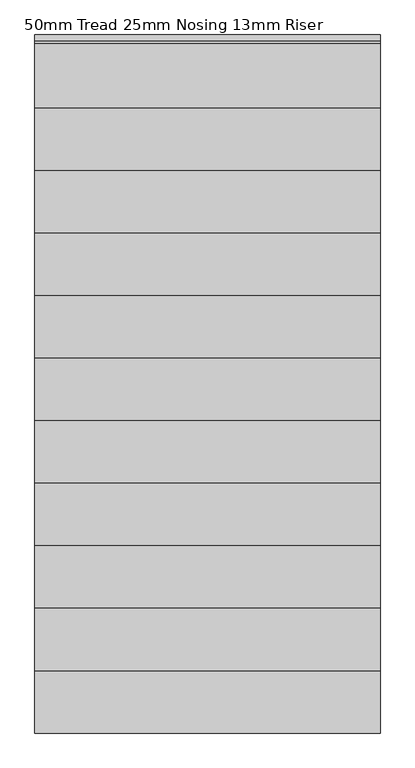
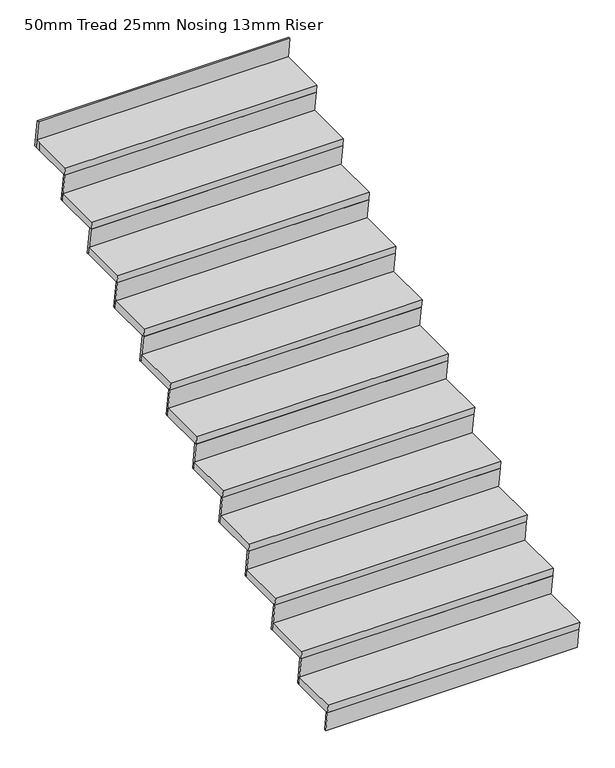
"""IFC4 building model written with IfcOpenShell, lengths in millimetres: stair flight geometry, 50mm Tread 25mm Nosing 13mm Riser."""

from ifc_helpers import new_model, si_unit, origin, place, context, project, spatial, faceted_brep, source, transform, mapped, element, save


def stair_flight_50mm_tread_25mm_nosing_13mm_riser_3e0063ee(model_context):
    return source(origin(), model_context, "Body", "Brep", [
        faceted_brep([(-499.4393676, 4584.7509075, 15676.4705882), (-499.4393676, 4591.8342409, 15626.4705882), (-2019.4393676, 4591.8342409, 15626.4705882), (-2019.4393676, 4584.7509075, 15676.4705882), (-2019.4393676, 4284.7509075, 15676.4705882), (-499.4393676, 4284.7509075, 15676.4705882), (-499.4393676, 4291.8342409, 15626.4705882), (-2019.4393676, 4291.8342409, 15626.4705882)], [[[0, 1, 2, 3]], [[3, 4, 5, 0]], [[2, 1, 6, 7]], [[4, 3, 2, 7]], [[0, 5, 6, 1]], [[5, 4, 7, 6]]]),
        faceted_brep([(-499.4393676, 4291.8342409, 15626.4705882), (-499.4393676, 4309.7509075, 15500.0), (-499.4393676, 4322.3757185, 15500.0), (-499.4393676, 4304.4590518, 15626.4705882), (-2019.4393676, 4291.8342409, 15626.4705882), (-2019.4393676, 4304.4590518, 15626.4705882), (-2019.4393676, 4322.3757185, 15500.0), (-2019.4393676, 4309.7509075, 15500.0)], [[[0, 1, 2, 3]], [[4, 5, 6, 7]], [[1, 0, 4, 7]], [[2, 1, 7, 6]], [[3, 2, 6, 5]], [[0, 3, 5, 4]]]),
        faceted_brep([(-499.4393676, 4566.8342409, 15802.9411765), (-499.4393676, 4591.8342409, 15626.4705882), (-499.4393676, 4604.4590518, 15626.4705882), (-499.4393676, 4579.4590518, 15802.9411765), (-2019.4393676, 4566.8342409, 15802.9411765), (-2019.4393676, 4579.4590518, 15802.9411765), (-2019.4393676, 4604.4590518, 15626.4705882), (-2019.4393676, 4591.8342409, 15626.4705882)], [[[0, 1, 2, 3]], [[4, 5, 6, 7]], [[1, 0, 4, 7]], [[2, 1, 7, 6]], [[3, 2, 6, 5]], [[0, 3, 5, 4]]]),
        faceted_brep([(-2019.4393676, 4859.7509075, 15852.9411765), (-2019.4393676, 4559.7509075, 15852.9411765), (-499.4393676, 4559.7509075, 15852.9411765), (-499.4393676, 4859.7509075, 15852.9411765), (-2019.4393676, 4866.8342409, 15802.9411765), (-499.4393676, 4866.8342409, 15802.9411765), (-499.4393676, 4566.8342409, 15802.9411765), (-2019.4393676, 4566.8342409, 15802.9411765)], [[[0, 1, 2, 3]], [[4, 5, 6, 7]], [[1, 0, 4, 7]], [[3, 2, 6, 5]], [[3, 5, 4, 0]], [[2, 1, 7, 6]]]),
        faceted_brep([(-499.4393676, 4841.8342409, 15979.4117647), (-499.4393676, 4866.8342409, 15802.9411765), (-499.4393676, 4879.4590518, 15802.9411765), (-499.4393676, 4854.4590518, 15979.4117647), (-2019.4393676, 4841.8342409, 15979.4117647), (-2019.4393676, 4854.4590518, 15979.4117647), (-2019.4393676, 4879.4590518, 15802.9411765), (-2019.4393676, 4866.8342409, 15802.9411765)], [[[0, 1, 2, 3]], [[4, 5, 6, 7]], [[1, 0, 4, 7]], [[2, 1, 7, 6]], [[3, 2, 6, 5]], [[0, 3, 5, 4]]]),
        faceted_brep([(-2019.4393676, 5134.7509075, 16029.4117647), (-2019.4393676, 4834.7509075, 16029.4117647), (-499.4393676, 4834.7509075, 16029.4117647), (-499.4393676, 5134.7509075, 16029.4117647), (-2019.4393676, 5141.8342409, 15979.4117647), (-499.4393676, 5141.8342409, 15979.4117647), (-499.4393676, 4841.8342409, 15979.4117647), (-2019.4393676, 4841.8342409, 15979.4117647)], [[[0, 1, 2, 3]], [[4, 5, 6, 7]], [[1, 0, 4, 7]], [[3, 2, 6, 5]], [[3, 5, 4, 0]], [[2, 1, 7, 6]]]),
        faceted_brep([(-499.4393676, 5116.8342409, 16155.8823529), (-499.4393676, 5141.8342409, 15979.4117647), (-499.4393676, 5154.4590518, 15979.4117647), (-499.4393676, 5129.4590518, 16155.8823529), (-2019.4393676, 5116.8342409, 16155.8823529), (-2019.4393676, 5129.4590518, 16155.8823529), (-2019.4393676, 5154.4590518, 15979.4117647), (-2019.4393676, 5141.8342409, 15979.4117647)], [[[0, 1, 2, 3]], [[4, 5, 6, 7]], [[1, 0, 4, 7]], [[2, 1, 7, 6]], [[3, 2, 6, 5]], [[0, 3, 5, 4]]]),
        faceted_brep([(-2019.4393676, 5409.7509075, 16205.8823529), (-2019.4393676, 5109.7509075, 16205.8823529), (-499.4393676, 5109.7509075, 16205.8823529), (-499.4393676, 5409.7509075, 16205.8823529), (-2019.4393676, 5416.8342409, 16155.8823529), (-499.4393676, 5416.8342409, 16155.8823529), (-499.4393676, 5116.8342409, 16155.8823529), (-2019.4393676, 5116.8342409, 16155.8823529)], [[[0, 1, 2, 3]], [[4, 5, 6, 7]], [[1, 0, 4, 7]], [[3, 2, 6, 5]], [[3, 5, 4, 0]], [[2, 1, 7, 6]]]),
        faceted_brep([(-499.4393676, 5391.8342409, 16332.3529412), (-499.4393676, 5416.8342409, 16155.8823529), (-499.4393676, 5429.4590518, 16155.8823529), (-499.4393676, 5404.4590518, 16332.3529412), (-2019.4393676, 5391.8342409, 16332.3529412), (-2019.4393676, 5404.4590518, 16332.3529412), (-2019.4393676, 5429.4590518, 16155.8823529), (-2019.4393676, 5416.8342409, 16155.8823529)], [[[0, 1, 2, 3]], [[4, 5, 6, 7]], [[1, 0, 4, 7]], [[2, 1, 7, 6]], [[3, 2, 6, 5]], [[0, 3, 5, 4]]]),
        faceted_brep([(-2019.4393676, 5684.7509075, 16382.3529412), (-2019.4393676, 5384.7509075, 16382.3529412), (-499.4393676, 5384.7509075, 16382.3529412), (-499.4393676, 5684.7509075, 16382.3529412), (-2019.4393676, 5691.8342409, 16332.3529412), (-499.4393676, 5691.8342409, 16332.3529412), (-499.4393676, 5391.8342409, 16332.3529412), (-2019.4393676, 5391.8342409, 16332.3529412)], [[[0, 1, 2, 3]], [[4, 5, 6, 7]], [[1, 0, 4, 7]], [[3, 2, 6, 5]], [[3, 5, 4, 0]], [[2, 1, 7, 6]]]),
        faceted_brep([(-499.4393676, 5666.8342409, 16508.8235294), (-499.4393676, 5691.8342409, 16332.3529412), (-499.4393676, 5704.4590518, 16332.3529412), (-499.4393676, 5679.4590518, 16508.8235294), (-2019.4393676, 5666.8342409, 16508.8235294), (-2019.4393676, 5679.4590518, 16508.8235294), (-2019.4393676, 5704.4590518, 16332.3529412), (-2019.4393676, 5691.8342409, 16332.3529412)], [[[0, 1, 2, 3]], [[4, 5, 6, 7]], [[1, 0, 4, 7]], [[2, 1, 7, 6]], [[3, 2, 6, 5]], [[0, 3, 5, 4]]]),
        faceted_brep([(-2019.4393676, 5959.7509075, 16558.8235294), (-2019.4393676, 5659.7509075, 16558.8235294), (-499.4393676, 5659.7509075, 16558.8235294), (-499.4393676, 5959.7509075, 16558.8235294), (-2019.4393676, 5966.8342409, 16508.8235294), (-499.4393676, 5966.8342409, 16508.8235294), (-499.4393676, 5666.8342409, 16508.8235294), (-2019.4393676, 5666.8342409, 16508.8235294)], [[[0, 1, 2, 3]], [[4, 5, 6, 7]], [[1, 0, 4, 7]], [[3, 2, 6, 5]], [[3, 5, 4, 0]], [[2, 1, 7, 6]]]),
        faceted_brep([(-499.4393676, 5941.8342409, 16685.2941176), (-499.4393676, 5966.8342409, 16508.8235294), (-499.4393676, 5979.4590518, 16508.8235294), (-499.4393676, 5954.4590518, 16685.2941176), (-2019.4393676, 5941.8342409, 16685.2941176), (-2019.4393676, 5954.4590518, 16685.2941176), (-2019.4393676, 5979.4590518, 16508.8235294), (-2019.4393676, 5966.8342409, 16508.8235294)], [[[0, 1, 2, 3]], [[4, 5, 6, 7]], [[1, 0, 4, 7]], [[2, 1, 7, 6]], [[3, 2, 6, 5]], [[0, 3, 5, 4]]]),
        faceted_brep([(-2019.4393676, 6234.7509075, 16735.2941176), (-2019.4393676, 5934.7509075, 16735.2941176), (-499.4393676, 5934.7509075, 16735.2941176), (-499.4393676, 6234.7509075, 16735.2941176), (-2019.4393676, 6241.8342409, 16685.2941176), (-499.4393676, 6241.8342409, 16685.2941176), (-499.4393676, 5941.8342409, 16685.2941176), (-2019.4393676, 5941.8342409, 16685.2941176)], [[[0, 1, 2, 3]], [[4, 5, 6, 7]], [[1, 0, 4, 7]], [[3, 2, 6, 5]], [[3, 5, 4, 0]], [[2, 1, 7, 6]]]),
        faceted_brep([(-499.4393676, 6216.8342409, 16861.7647059), (-499.4393676, 6241.8342409, 16685.2941176), (-499.4393676, 6254.4590518, 16685.2941176), (-499.4393676, 6229.4590518, 16861.7647059), (-2019.4393676, 6216.8342409, 16861.7647059), (-2019.4393676, 6229.4590518, 16861.7647059), (-2019.4393676, 6254.4590518, 16685.2941176), (-2019.4393676, 6241.8342409, 16685.2941176)], [[[0, 1, 2, 3]], [[4, 5, 6, 7]], [[1, 0, 4, 7]], [[2, 1, 7, 6]], [[3, 2, 6, 5]], [[0, 3, 5, 4]]]),
        faceted_brep([(-2019.4393676, 6509.7509075, 16911.7647059), (-2019.4393676, 6209.7509075, 16911.7647059), (-499.4393676, 6209.7509075, 16911.7647059), (-499.4393676, 6509.7509075, 16911.7647059), (-2019.4393676, 6516.8342409, 16861.7647059), (-499.4393676, 6516.8342409, 16861.7647059), (-499.4393676, 6216.8342409, 16861.7647059), (-2019.4393676, 6216.8342409, 16861.7647059)], [[[0, 1, 2, 3]], [[4, 5, 6, 7]], [[1, 0, 4, 7]], [[3, 2, 6, 5]], [[3, 5, 4, 0]], [[2, 1, 7, 6]]]),
        faceted_brep([(-499.4393676, 6491.8342409, 17038.2352941), (-499.4393676, 6516.8342409, 16861.7647059), (-499.4393676, 6529.4590518, 16861.7647059), (-499.4393676, 6504.4590518, 17038.2352941), (-2019.4393676, 6491.8342409, 17038.2352941), (-2019.4393676, 6504.4590518, 17038.2352941), (-2019.4393676, 6529.4590518, 16861.7647059), (-2019.4393676, 6516.8342409, 16861.7647059)], [[[0, 1, 2, 3]], [[4, 5, 6, 7]], [[1, 0, 4, 7]], [[2, 1, 7, 6]], [[3, 2, 6, 5]], [[0, 3, 5, 4]]]),
        faceted_brep([(-2019.4393676, 6784.7509075, 17088.2352941), (-2019.4393676, 6484.7509075, 17088.2352941), (-499.4393676, 6484.7509075, 17088.2352941), (-499.4393676, 6784.7509075, 17088.2352941), (-2019.4393676, 6791.8342409, 17038.2352941), (-499.4393676, 6791.8342409, 17038.2352941), (-499.4393676, 6491.8342409, 17038.2352941), (-2019.4393676, 6491.8342409, 17038.2352941)], [[[0, 1, 2, 3]], [[4, 5, 6, 7]], [[1, 0, 4, 7]], [[3, 2, 6, 5]], [[3, 5, 4, 0]], [[2, 1, 7, 6]]]),
        faceted_brep([(-499.4393676, 6766.8342409, 17214.7058824), (-499.4393676, 6791.8342409, 17038.2352941), (-499.4393676, 6804.4590518, 17038.2352941), (-499.4393676, 6779.4590518, 17214.7058824), (-2019.4393676, 6766.8342409, 17214.7058824), (-2019.4393676, 6779.4590518, 17214.7058824), (-2019.4393676, 6804.4590518, 17038.2352941), (-2019.4393676, 6791.8342409, 17038.2352941)], [[[0, 1, 2, 3]], [[4, 5, 6, 7]], [[1, 0, 4, 7]], [[2, 1, 7, 6]], [[3, 2, 6, 5]], [[0, 3, 5, 4]]]),
        faceted_brep([(-2019.4393676, 7059.7509075, 17264.7058824), (-2019.4393676, 6759.7509075, 17264.7058824), (-499.4393676, 6759.7509075, 17264.7058824), (-499.4393676, 7059.7509075, 17264.7058824), (-2019.4393676, 7066.8342409, 17214.7058824), (-499.4393676, 7066.8342409, 17214.7058824), (-499.4393676, 6766.8342409, 17214.7058824), (-2019.4393676, 6766.8342409, 17214.7058824)], [[[0, 1, 2, 3]], [[4, 5, 6, 7]], [[1, 0, 4, 7]], [[3, 2, 6, 5]], [[3, 5, 4, 0]], [[2, 1, 7, 6]]]),
        faceted_brep([(-499.4393676, 7316.8342409, 17567.6470588), (-499.4393676, 7341.8342409, 17391.1764706), (-499.4393676, 7354.4590518, 17391.1764706), (-499.4393676, 7329.4590518, 17567.6470588), (-2019.4393676, 7316.8342409, 17567.6470588), (-2019.4393676, 7329.4590518, 17567.6470588), (-2019.4393676, 7354.4590518, 17391.1764706), (-2019.4393676, 7341.8342409, 17391.1764706)], [[[0, 1, 2, 3]], [[4, 5, 6, 7]], [[1, 0, 4, 7]], [[2, 1, 7, 6]], [[3, 2, 6, 5]], [[0, 3, 5, 4]]]),
        faceted_brep([(-499.4393676, 7041.8342409, 17391.1764706), (-499.4393676, 7066.8342409, 17214.7058824), (-499.4393676, 7079.4590518, 17214.7058824), (-499.4393676, 7054.4590518, 17391.1764706), (-2019.4393676, 7041.8342409, 17391.1764706), (-2019.4393676, 7054.4590518, 17391.1764706), (-2019.4393676, 7079.4590518, 17214.7058824), (-2019.4393676, 7066.8342409, 17214.7058824)], [[[0, 1, 2, 3]], [[4, 5, 6, 7]], [[1, 0, 4, 7]], [[2, 1, 7, 6]], [[3, 2, 6, 5]], [[0, 3, 5, 4]]]),
        faceted_brep([(-2019.4393676, 7334.7509075, 17441.1764706), (-2019.4393676, 7309.7509075, 17441.1764706), (-2019.4393676, 7034.7509075, 17441.1764706), (-499.4393676, 7034.7509075, 17441.1764706), (-499.4393676, 7334.7509075, 17441.1764706), (-2019.4393676, 7341.8342409, 17391.1764706), (-499.4393676, 7341.8342409, 17391.1764706), (-499.4393676, 7041.8342409, 17391.1764706), (-2019.4393676, 7041.8342409, 17391.1764706), (-2019.4393676, 7309.7509075, 17391.1764706)], [[[0, 1, 2, 3, 4]], [[5, 6, 7, 8, 9]], [[1, 0, 5, 9]], [[2, 1, 9, 8]], [[4, 3, 7, 6]], [[4, 6, 5, 0]], [[3, 2, 8, 7]]]),
    ])


if __name__ == "__main__":
    model = new_model("IFC4")
    model_context = context("Model", 3, world=origin())
    ifc_project = project(units=[si_unit("LENGTHUNIT", "METRE", prefix="MILLI")], contexts=[model_context])
    site = spatial("IfcSite", under=ifc_project)
    building = spatial("IfcBuilding", under=site)
    placement = place(None, origin())
    stair_flight_50mm_tread_25mm_nosing_13mm_riser_shape = stair_flight_50mm_tread_25mm_nosing_13mm_riser_3e0063ee(model_context)
    element("IfcStairFlight", 1, ObjectType="50mm Tread 25mm Nosing 13mm Riser", at=placement, inside=building, context=model_context, shape_type="MappedRepresentation", body=[
        mapped(stair_flight_50mm_tread_25mm_nosing_13mm_riser_shape, transform((0.0, 0.0, 0.0), x_axis=(1.0, 0.0, 0.0), y_axis=(0.0, 1.0, 0.0), z_axis=(0.0, 0.0, 1.0))),
    ])
    save(model, "model.ifc")
